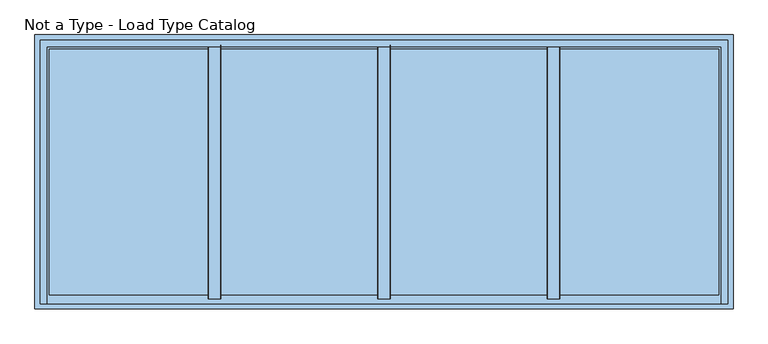
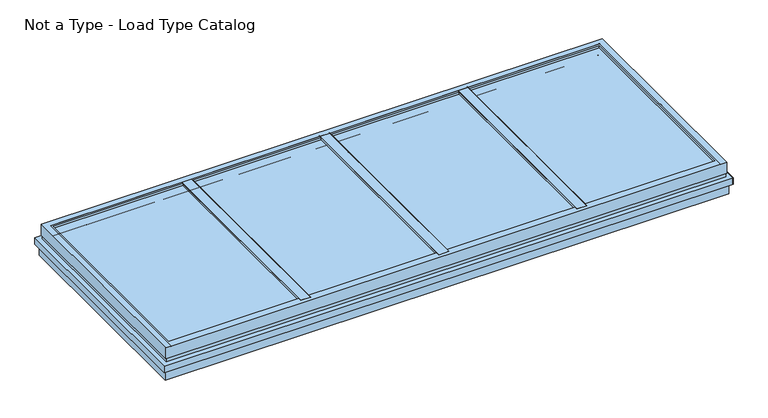
"""IFC4 building model written with IfcOpenShell, lengths in millimetres: window geometry, Skylight-Wasco-Low_Profile : Not a Type - Load Type Catalog."""

from ifc_helpers import new_model, si_unit, point, frame, frame_2d, origin, origin_with_axes, place, context, project, spatial, polyline, circle_curve, ellipse_curve, trimmed, segment, composite_curve, outline, extrude, source, transform, mapped, element, save
from ifc_brep_helpers import plane_surface, cylinder_surface, advanced_brep


def not_a_type_load_type_catalog_e0b292cc(model_context):
    return source(origin(), model_context, "Body", "SolidModel", [
        extrude(outline(composite_curve([segment(polyline([(192.3802188, 28.1940003), (192.3802188, -28.1940003)]), True, "CONTINUOUS"), segment(trimmed(circle_curve(frame_2d((178.9315699, -28.1940003)), 13.4486489), [point((192.3802188, -28.1940003))], [point((192.2262471, -30.2232155))], False, "CARTESIAN"), True, "CONTINUOUS"), segment(polyline([(192.2262471, -30.2232155), (179.4099406, -29.6347387), (179.4099406, -26.7462003), (176.2344841, -26.7462003), (176.2344841, -9.5227863), (142.8969841, -9.5227863), (142.8969841, -22.2249447), (139.7215663, -22.2249447), (139.7215663, -26.924), (138.1213663, -26.924), (136.5948503, -25.4), (111.715375, -25.4)]), True, "CONTINUOUS"), segment(trimmed(circle_curve(frame_2d((111.715375, -28.575)), 3.175), [point((111.715375, -25.4))], [point((108.5468841, -28.7782))], True, "CARTESIAN"), True, "CONTINUOUS"), segment(trimmed(circle_curve(frame_2d((111.715375, -28.9814)), 3.175), [point((108.5468841, -28.7782))], [point((111.715375, -32.1564))], True, "CARTESIAN"), True, "CONTINUOUS"), segment(polyline([(111.715375, -32.1564), (116.683615, -32.1564)]), True, "CONTINUOUS"), segment(trimmed(circle_curve(frame_2d((116.683615, -33.5407)), 1.3843), [point((116.683615, -32.1564))], [point((116.683615, -34.925))], False, "CARTESIAN"), True, "CONTINUOUS"), segment(polyline([(116.683615, -34.925), (101.6, -34.925), (101.6, 34.925), (116.683615, 34.925)]), True, "CONTINUOUS"), segment(trimmed(circle_curve(frame_2d((116.683615, 33.5407)), 1.3843), [point((116.683615, 34.925))], [point((116.683615, 32.1564))], False, "CARTESIAN"), True, "CONTINUOUS"), segment(polyline([(116.683615, 32.1564), (111.715375, 32.1564)]), True, "CONTINUOUS"), segment(trimmed(circle_curve(frame_2d((111.715375, 28.9814)), 3.175), [point((111.715375, 32.1564))], [point((108.5468841, 28.7782))], True, "CARTESIAN"), True, "CONTINUOUS"), segment(trimmed(circle_curve(frame_2d((111.715375, 28.575)), 3.175), [point((108.5468841, 28.7782))], [point((111.715375, 25.4))], True, "CARTESIAN"), True, "CONTINUOUS"), segment(polyline([(111.715375, 25.4), (136.5948503, 25.4), (138.1213663, 26.924), (139.7215663, 26.924), (139.7215663, 22.2249447), (142.8969841, 22.2249447), (142.8969841, 9.5227863), (176.2344841, 9.5227863), (176.2344841, 26.7462003), (179.4099406, 26.7462003), (179.4099406, 29.6347387), (190.2418721, 30.2232155)]), True, "CONTINUOUS"), segment(trimmed(circle_curve(frame_2d((190.3482188, 28.1940003)), 2.032), [point((190.2418721, 30.2232155))], [point((192.3802188, 28.1940003))], False, "CARTESIAN"), True, "CONTINUOUS")], self_intersect=False)), frame((0.0, -609.6, 0.0), z_axis=(0.0, 1.0, 0.0), x_axis=(0.0, 0.0, 1.0)), (0.0, 0.0, 1.0), 1219.2),
        extrude(outline(polyline([(25.4, -609.6), (-25.4, -609.6), (-25.4, 609.6), (25.4, 609.6), (25.4, -609.6)])), frame((0.0, 0.0, 0.3569904), z_axis=(0.0, 0.0, 1.0), x_axis=(1.0, 0.0, 0.0)), (0.0, 0.0, 1.0), 100.80625),
        extrude(outline(composite_curve([segment(polyline([(192.3802188, -784.6059997), (192.3802188, -840.9940003)]), True, "CONTINUOUS"), segment(trimmed(circle_curve(frame_2d((178.9315699, -840.9940003)), 13.4486489), [point((192.3802188, -840.9940003))], [point((192.2262471, -843.0232155))], False, "CARTESIAN"), True, "CONTINUOUS"), segment(polyline([(192.2262471, -843.0232155), (179.4099406, -842.4347387), (179.4099406, -839.5462003), (176.2344841, -839.5462003), (176.2344841, -822.3227863), (142.8969841, -822.3227863), (142.8969841, -835.0249447), (139.7215663, -835.0249447), (139.7215663, -839.724), (138.1213663, -839.724), (136.5948503, -838.2), (111.715375, -838.2)]), True, "CONTINUOUS"), segment(trimmed(circle_curve(frame_2d((111.715375, -841.375)), 3.175), [point((111.715375, -838.2))], [point((108.5468841, -841.5782))], True, "CARTESIAN"), True, "CONTINUOUS"), segment(trimmed(circle_curve(frame_2d((111.715375, -841.7814)), 3.175), [point((108.5468841, -841.5782))], [point((111.715375, -844.9564))], True, "CARTESIAN"), True, "CONTINUOUS"), segment(polyline([(111.715375, -844.9564), (116.683615, -844.9564)]), True, "CONTINUOUS"), segment(trimmed(circle_curve(frame_2d((116.683615, -846.3407)), 1.3843), [point((116.683615, -844.9564))], [point((116.683615, -847.725))], False, "CARTESIAN"), True, "CONTINUOUS"), segment(polyline([(116.683615, -847.725), (101.6, -847.725), (101.6, -777.875), (116.683615, -777.875)]), True, "CONTINUOUS"), segment(trimmed(circle_curve(frame_2d((116.683615, -779.2593)), 1.3843), [point((116.683615, -777.875))], [point((116.683615, -780.6436))], False, "CARTESIAN"), True, "CONTINUOUS"), segment(polyline([(116.683615, -780.6436), (111.715375, -780.6436)]), True, "CONTINUOUS"), segment(trimmed(circle_curve(frame_2d((111.715375, -783.8186)), 3.175), [point((111.715375, -780.6436))], [point((108.5468841, -784.0218))], True, "CARTESIAN"), True, "CONTINUOUS"), segment(trimmed(circle_curve(frame_2d((111.715375, -784.225)), 3.175), [point((108.5468841, -784.0218))], [point((111.715375, -787.4))], True, "CARTESIAN"), True, "CONTINUOUS"), segment(polyline([(111.715375, -787.4), (136.5948503, -787.4), (138.1213663, -785.876), (139.7215663, -785.876), (139.7215663, -790.5750553), (142.8969841, -790.5750553), (142.8969841, -803.2772137), (176.2344841, -803.2772137), (176.2344841, -786.0537997), (179.4099406, -786.0537997), (179.4099406, -783.1652613), (190.2418721, -782.5767845)]), True, "CONTINUOUS"), segment(trimmed(circle_curve(frame_2d((190.3482188, -784.6059997)), 2.032), [point((190.2418721, -782.5767845))], [point((192.3802188, -784.6059997))], False, "CARTESIAN"), True, "CONTINUOUS")], self_intersect=False)), frame((0.0, -609.6, 0.0), z_axis=(0.0, 1.0, 0.0), x_axis=(0.0, 0.0, 1.0)), (0.0, 0.0, 1.0), 1219.2),
        extrude(outline(polyline([(-787.4, -609.6), (-838.2, -609.6), (-838.2, 609.6), (-787.4, 609.6), (-787.4, -609.6)])), frame((0.0, 0.0, 0.3569904), z_axis=(0.0, 0.0, 1.0), x_axis=(1.0, 0.0, 0.0)), (0.0, 0.0, 1.0), 100.80625),
        extrude(outline(composite_curve([segment(polyline([(192.3802188, 840.9940003), (192.3802188, 784.6059997)]), True, "CONTINUOUS"), segment(trimmed(circle_curve(frame_2d((178.9315699, 784.6059997)), 13.4486489), [point((192.3802188, 784.6059997))], [point((192.2262471, 782.5767845))], False, "CARTESIAN"), True, "CONTINUOUS"), segment(polyline([(192.2262471, 782.5767845), (179.4099406, 783.1652613), (179.4099406, 786.0537997), (176.2344841, 786.0537997), (176.2344841, 803.2772137), (142.8969841, 803.2772137), (142.8969841, 790.5750553), (139.7215663, 790.5750553), (139.7215663, 785.876), (138.1213663, 785.876), (136.5948503, 787.4), (111.715375, 787.4)]), True, "CONTINUOUS"), segment(trimmed(circle_curve(frame_2d((111.715375, 784.225)), 3.175), [point((111.715375, 787.4))], [point((108.5468841, 784.0218))], True, "CARTESIAN"), True, "CONTINUOUS"), segment(trimmed(circle_curve(frame_2d((111.715375, 783.8186)), 3.175), [point((108.5468841, 784.0218))], [point((111.715375, 780.6436))], True, "CARTESIAN"), True, "CONTINUOUS"), segment(polyline([(111.715375, 780.6436), (116.683615, 780.6436)]), True, "CONTINUOUS"), segment(trimmed(circle_curve(frame_2d((116.683615, 779.2593)), 1.3843), [point((116.683615, 780.6436))], [point((116.683615, 777.875))], False, "CARTESIAN"), True, "CONTINUOUS"), segment(polyline([(116.683615, 777.875), (101.6, 777.875), (101.6, 847.725), (116.683615, 847.725)]), True, "CONTINUOUS"), segment(trimmed(circle_curve(frame_2d((116.683615, 846.3407)), 1.3843), [point((116.683615, 847.725))], [point((116.683615, 844.9564))], False, "CARTESIAN"), True, "CONTINUOUS"), segment(polyline([(116.683615, 844.9564), (111.715375, 844.9564)]), True, "CONTINUOUS"), segment(trimmed(circle_curve(frame_2d((111.715375, 841.7814)), 3.175), [point((111.715375, 844.9564))], [point((108.5468841, 841.5782))], True, "CARTESIAN"), True, "CONTINUOUS"), segment(trimmed(circle_curve(frame_2d((111.715375, 841.375)), 3.175), [point((108.5468841, 841.5782))], [point((111.715375, 838.2))], True, "CARTESIAN"), True, "CONTINUOUS"), segment(polyline([(111.715375, 838.2), (136.5948503, 838.2), (138.1213663, 839.724), (139.7215663, 839.724), (139.7215663, 835.0249447), (142.8969841, 835.0249447), (142.8969841, 822.3227863), (176.2344841, 822.3227863), (176.2344841, 839.5462003), (179.4099406, 839.5462003), (179.4099406, 842.4347387), (190.2418721, 843.0232155)]), True, "CONTINUOUS"), segment(trimmed(circle_curve(frame_2d((190.3482188, 840.9940003)), 2.032), [point((190.2418721, 843.0232155))], [point((192.3802188, 840.9940003))], False, "CARTESIAN"), True, "CONTINUOUS")], self_intersect=False)), frame((0.0, -609.6, 0.0), z_axis=(0.0, 1.0, 0.0), x_axis=(0.0, 0.0, 1.0)), (0.0, 0.0, 1.0), 1219.2),
        extrude(outline(polyline([(838.2, -609.6), (787.4, -609.6), (787.4, 609.6), (838.2, 609.6), (838.2, -609.6)])), frame((0.0, 0.0, 0.3569904), z_axis=(0.0, 0.0, 1.0), x_axis=(1.0, 0.0, 0.0)), (0.0, 0.0, 1.0), 100.80625),
        advanced_brep(
        [(-1603.6480651, -587.6480651, 136.468788), (-1607.2040651, -591.2040651, 132.912788), (-1607.2040651, 591.2040651, 132.912788), (-1603.6480651, 587.6480651, 136.468788), (-1603.6480651, 587.6480651, 146.0493661), (-1603.6480651, -587.6480651, 146.0493661), (-1617.109615, 601.109615, 192.469164), (-1617.109615, 601.109615, 193.8734375), (-1617.109615, -633.6302051, 193.8734375), (-1617.109615, -633.6302051, 192.469164), (-1594.8851432, -578.8851432, 117.475), (-1594.1231432, -578.1231432, 116.713), (-1594.1231432, 578.1231432, 116.713), (-1594.8851432, 578.8851432, 117.475), (-1672.1854051, -656.1854051, 101.6), (-1672.1854051, -656.1854051, 63.5), (-1672.1854051, 656.1854051, 63.5), (-1672.1854051, 656.1854051, 101.6), (-1674.2174051, -658.2174051, 63.5), (-1674.2174051, -658.2174051, 103.632), (-1674.2174051, 658.2174051, 103.632), (-1674.2174051, 658.2174051, 63.5), (-1606.55, -590.55, 192.469164), (-1606.55, -590.55, 179.3876533), (-1606.55, 590.55, 179.3876533), (-1606.55, 590.55, 192.469164), (-1622.3607127, -606.3607127, 179.3876533), (-1622.3607127, -606.3607127, 146.0493661), (-1622.3607127, 606.3607127, 146.0493661), (-1622.3607127, 606.3607127, 179.3876533), (-1612.3113821, -596.3113821, 132.912788), (-1612.3113821, -596.3113821, 117.475), (-1612.3113821, 596.3113821, 117.475), (-1612.3113821, 596.3113821, 132.912788), (-1594.1231432, -578.1231432, 101.6), (-1594.1231432, 578.1231432, 101.6), (-1646.4979432, -630.4979432, 103.632), (-1646.4979432, -630.4979432, 125.7990653), (-1646.4979432, 630.4979432, 125.7990653), (-1646.4979432, 630.4979432, 103.632), (-1649.6302051, -633.6302051, 125.7990653), (-1649.6302051, -633.6302051, 193.8734375), (-1649.6302051, 633.6302051, 193.8734375), (-1649.6302051, 633.6302051, 125.7990653), (1606.55, 590.55, 179.3876533), (1606.55, 590.55, 192.469164), (1622.3607127, 606.3607127, 146.0493661), (1622.3607127, 606.3607127, 179.3876533), (1612.3113821, 596.3113821, 117.475), (1612.3113821, 596.3113821, 132.912788), (1594.1231432, 578.1231432, 101.6), (1594.1231432, 578.1231432, 116.713), (1646.4979432, 630.4979432, 125.7990653), (1646.4979432, 630.4979432, 103.632), (1649.6302051, 633.6302051, 193.8734375), (1649.6302051, 633.6302051, 125.7990653), (1606.55, -590.55, 179.3876533), (1606.55, -590.55, 192.469164), (1622.3607127, -606.3607127, 146.0493661), (1622.3607127, -606.3607127, 179.3876533), (1612.3113821, -596.3113821, 117.475), (1612.3113821, -596.3113821, 132.912788), (1594.1231432, -578.1231432, 101.6), (1594.1231432, -578.1231432, 116.713), (1646.4979432, -630.4979432, 125.7990653), (1646.4979432, -630.4979432, 103.632), (1649.6302051, -633.6302051, 193.8734375), (1649.6302051, -633.6302051, 125.7990653), (1594.8851432, 578.8851432, 117.475), (1607.2040651, 591.2040651, 132.912788), (1603.6480651, 587.6480651, 136.468788), (1603.6480651, 587.6480651, 146.0493661), (1617.109615, 601.109615, 192.469164), (1617.109615, 601.109615, 193.8734375), (1594.8851432, -578.8851432, 117.475), (1607.2040651, -591.2040651, 132.912788), (1603.6480651, -587.6480651, 136.468788), (1603.6480651, -587.6480651, 146.0493661), (1617.109615, -633.6302051, 192.469164), (1617.109615, -633.6302051, 193.8734375), (1672.1854051, 656.1854051, 101.6), (1672.1854051, -656.1854051, 101.6), (1674.2174051, 658.2174051, 103.632), (1674.2174051, 658.2174051, 63.5), (1672.1854051, 656.1854051, 63.5), (1674.2174051, -658.2174051, 103.632), (1674.2174051, -658.2174051, 63.5), (1672.1854051, -656.1854051, 63.5)],
        [
            (0, 1, ellipse_curve(frame((-1607.2040651, -591.2040651, 136.468788), z_axis=(-0.7071067811865475, 0.7071067811865475, 0.0), x_axis=(-0.7071067811865474, -0.7071067811865476, 0.0)), 5.0289434, 3.556)),
            (1, 2),
            (2, 3, ellipse_curve(frame((-1607.2040651, 591.2040651, 136.468788), z_axis=(-0.7071067811865475, -0.7071067811865475, 0.0), x_axis=(0.7071067811865474, -0.7071067811865476, 0.0)), 5.0289434, 3.556)),
            (3, 0),
            (3, 4),
            (4, 5),
            (5, 0),
            (6, 7),
            (7, 8),
            (8, 9),
            (9, 6),
            (10, 11, ellipse_curve(frame((-1594.8851432, -578.8851432, 116.713), z_axis=(-0.7071067811865475, 0.7071067811865475, 0.0), x_axis=(-0.7071067811865474, -0.7071067811865476, 0.0)), 1.0776307, 0.762)),
            (11, 12),
            (12, 13, ellipse_curve(frame((-1594.8851432, 578.8851432, 116.713), z_axis=(-0.7071067811865475, -0.7071067811865475, 0.0), x_axis=(0.7071067811865474, -0.7071067811865476, 0.0)), 1.0776307, 0.762)),
            (13, 10),
            (14, 15),
            (15, 16),
            (16, 17),
            (17, 14),
            (18, 19),
            (19, 20),
            (20, 21),
            (21, 18),
            (22, 23),
            (23, 24),
            (24, 25),
            (25, 22),
            (26, 27),
            (27, 28),
            (28, 29),
            (29, 26),
            (30, 31),
            (31, 32),
            (32, 33),
            (33, 30),
            (11, 34),
            (34, 35),
            (35, 12),
            (36, 37),
            (37, 38),
            (38, 39),
            (39, 36),
            (40, 41),
            (41, 42),
            (42, 43),
            (43, 40),
            (24, 44),
            (44, 45),
            (45, 25),
            (28, 46),
            (46, 47),
            (47, 29),
            (32, 48),
            (48, 49),
            (49, 33),
            (35, 50),
            (50, 51),
            (51, 12),
            (38, 52),
            (52, 53),
            (53, 39),
            (42, 54),
            (54, 55),
            (55, 43),
            (44, 56),
            (56, 57),
            (57, 45),
            (46, 58),
            (58, 59),
            (59, 47),
            (48, 60),
            (60, 61),
            (61, 49),
            (50, 62),
            (62, 63),
            (63, 51),
            (52, 64),
            (64, 65),
            (65, 53),
            (54, 66),
            (66, 67),
            (67, 55),
            (51, 68, ellipse_curve(frame((1594.8851432, 578.8851432, 116.713), z_axis=(-0.7071067811865475, 0.7071067811865475, 0.0), x_axis=(-0.7071067811865476, -0.7071067811865474, 0.0)), 1.0776307, 0.762)),
            (68, 13),
            (2, 69),
            (69, 70, ellipse_curve(frame((1607.2040651, 591.2040651, 136.468788), z_axis=(-0.7071067811865475, 0.7071067811865475, 0.0), x_axis=(-0.7071067811865476, -0.7071067811865474, 0.0)), 5.0289434, 3.556)),
            (70, 3),
            (70, 71),
            (71, 4),
            (6, 72),
            (72, 73),
            (73, 7),
            (63, 74, ellipse_curve(frame((1594.8851432, -578.8851432, 116.713), z_axis=(0.7071067811865475, 0.7071067811865475, 0.0), x_axis=(-0.7071067811865474, 0.7071067811865476, 0.0)), 1.0776307, 0.762)),
            (74, 68),
            (69, 75),
            (75, 76, ellipse_curve(frame((1607.2040651, -591.2040651, 136.468788), z_axis=(0.7071067811865475, 0.7071067811865475, 0.0), x_axis=(-0.7071067811865474, 0.7071067811865476, 0.0)), 5.0289434, 3.556)),
            (76, 70),
            (76, 77),
            (77, 71),
            (72, 78),
            (78, 79),
            (79, 73),
            (40, 67),
            (66, 79),
            (78, 9),
            (8, 41),
            (37, 64),
            (36, 65),
            (17, 80),
            (80, 81),
            (81, 14),
            (34, 62),
            (11, 63),
            (10, 74),
            (31, 60),
            (30, 61),
            (1, 75),
            (0, 76),
            (5, 77),
            (27, 58),
            (26, 59),
            (23, 56),
            (57, 22),
            (20, 82),
            (82, 83),
            (83, 21),
            (16, 84),
            (84, 80),
            (82, 85),
            (85, 86),
            (86, 83),
            (84, 87),
            (87, 81),
            (19, 85),
            (18, 86),
            (15, 87),
        ],
        [
            cylinder_surface(frame((-1607.2040651, -633.6302051, 136.468788), z_axis=(0.0, -1.0, 0.0), x_axis=(1.0, 0.0, 0.0)), 3.556),
            plane_surface(frame((-1603.6480651, -587.6480651, 136.468788), z_axis=(1.0, 0.0, 0.0), x_axis=(0.0, 1.0, 0.0))),
            plane_surface(frame((-1617.109615, -601.109615, 192.469164), z_axis=(1.0, 0.0, 0.0), x_axis=(0.0, 1.0, 0.0))),
            cylinder_surface(frame((-1594.8851432, -633.6302051, 116.713), z_axis=(0.0, -1.0, 0.0), x_axis=(1.0, 0.0, 0.0)), 0.762),
            plane_surface(frame((-1672.1854051, -656.1854051, 63.5), z_axis=(1.0, 0.0, 0.0), x_axis=(0.0, 1.0, 0.0))),
            plane_surface(frame((-1674.2174051, -658.2174051, 103.632), z_axis=(-1.0, 0.0, 0.0), x_axis=(0.0, 1.0, 0.0))),
            plane_surface(frame((-1606.55, -590.55, 179.3876533), z_axis=(1.0, 0.0, 0.0), x_axis=(0.0, 1.0, 0.0))),
            plane_surface(frame((-1622.3607127, -606.3607127, 146.0493661), z_axis=(1.0, 0.0, 0.0), x_axis=(0.0, 1.0, 0.0))),
            plane_surface(frame((-1612.3113821, -596.3113821, 117.475), z_axis=(1.0, 0.0, 0.0), x_axis=(0.0, 1.0, 0.0))),
            plane_surface(frame((-1594.1231432, -578.1231432, 101.6), z_axis=(1.0, 0.0, 0.0), x_axis=(0.0, 1.0, 0.0))),
            plane_surface(frame((-1646.4979432, -630.4979432, 125.7990653), z_axis=(-1.0, 0.0, 0.0), x_axis=(0.0, 1.0, 0.0))),
            plane_surface(frame((-1649.6302051, -633.6302051, 193.8734375), z_axis=(-1.0, 0.0, 0.0), x_axis=(0.0, 1.0, 0.0))),
            plane_surface(frame((-1606.55, 590.55, 179.3876533), z_axis=(0.0, -1.0, 0.0), x_axis=(1.0, 0.0, 0.0))),
            plane_surface(frame((-1622.3607127, 606.3607127, 146.0493661), z_axis=(0.0, -1.0, 0.0), x_axis=(1.0, 0.0, 0.0))),
            plane_surface(frame((-1612.3113821, 596.3113821, 117.475), z_axis=(0.0, -1.0, 0.0), x_axis=(1.0, 0.0, 0.0))),
            plane_surface(frame((-1594.1231432, 578.1231432, 101.6), z_axis=(0.0, -1.0, 0.0), x_axis=(1.0, 0.0, 0.0))),
            plane_surface(frame((-1646.4979432, 630.4979432, 125.7990653), z_axis=(0.0, 1.0, 0.0), x_axis=(1.0, 0.0, 0.0))),
            plane_surface(frame((-1649.6302051, 633.6302051, 193.8734375), z_axis=(0.0, 1.0, 0.0), x_axis=(1.0, 0.0, 0.0))),
            plane_surface(frame((1606.55, 590.55, 179.3876533), z_axis=(-1.0, 0.0, 0.0), x_axis=(0.0, -1.0, 0.0))),
            plane_surface(frame((1622.3607127, 606.3607127, 146.0493661), z_axis=(-1.0, 0.0, 0.0), x_axis=(0.0, -1.0, 0.0))),
            plane_surface(frame((1612.3113821, 596.3113821, 117.475), z_axis=(-1.0, 0.0, 0.0), x_axis=(0.0, -1.0, 0.0))),
            plane_surface(frame((1594.1231432, 578.1231432, 101.6), z_axis=(-1.0, 0.0, 0.0), x_axis=(0.0, -1.0, 0.0))),
            plane_surface(frame((1646.4979432, 630.4979432, 125.7990653), z_axis=(1.0, 0.0, 0.0), x_axis=(0.0, -1.0, 0.0))),
            plane_surface(frame((1649.6302051, 633.6302051, 193.8734375), z_axis=(1.0, 0.0, 0.0), x_axis=(0.0, -1.0, 0.0))),
            cylinder_surface(frame((-1649.6302051, 578.8851432, 116.713), z_axis=(-1.0, 0.0, 0.0), x_axis=(0.0, -1.0, 0.0)), 0.762),
            cylinder_surface(frame((-1649.6302051, 591.2040651, 136.468788), z_axis=(-1.0, 0.0, 0.0), x_axis=(0.0, -1.0, 0.0)), 3.556),
            plane_surface(frame((-1603.6480651, 587.6480651, 136.468788), z_axis=(0.0, -1.0, 0.0), x_axis=(1.0, 0.0, 0.0))),
            plane_surface(frame((-1617.109615, 601.109615, 192.469164), z_axis=(0.0, -1.0, 0.0), x_axis=(1.0, 0.0, 0.0))),
            cylinder_surface(frame((1594.8851432, 633.6302051, 116.713), z_axis=(0.0, 1.0, 0.0), x_axis=(-1.0, 0.0, 0.0)), 0.762),
            cylinder_surface(frame((1607.2040651, 633.6302051, 136.468788), z_axis=(0.0, 1.0, 0.0), x_axis=(-1.0, 0.0, 0.0)), 3.556),
            plane_surface(frame((1603.6480651, 587.6480651, 136.468788), z_axis=(-1.0, 0.0, 0.0), x_axis=(0.0, -1.0, 0.0))),
            plane_surface(frame((1617.109615, 601.109615, 192.469164), z_axis=(-1.0, 0.0, 0.0), x_axis=(0.0, -1.0, 0.0))),
            plane_surface(frame((1649.6302051, -633.6302051, 193.8734375), z_axis=(0.0, -1.0, 0.0), x_axis=(-1.0, 0.0, 0.0))),
            plane_surface(frame((1649.6302051, -633.6302051, 125.7990653), z_axis=(0.0, 0.0, -1.0), x_axis=(-1.0, 0.0, 0.0))),
            plane_surface(frame((1646.4979432, -630.4979432, 125.7990653), z_axis=(0.0, -1.0, 0.0), x_axis=(-1.0, 0.0, 0.0))),
            plane_surface(frame((1672.1854051, -656.1854051, 101.6), z_axis=(0.0, 0.0, -1.0), x_axis=(-1.0, 0.0, 0.0))),
            plane_surface(frame((1594.1231432, -578.1231432, 101.6), z_axis=(0.0, 1.0, 0.0), x_axis=(-1.0, 0.0, 0.0))),
            cylinder_surface(frame((1649.6302051, -578.8851432, 116.713), z_axis=(1.0, 0.0, 0.0), x_axis=(0.0, 1.0, 0.0)), 0.762),
            plane_surface(frame((1594.8851432, -578.8851432, 117.475), z_axis=(0.0, 0.0, 1.0), x_axis=(-1.0, 0.0, 0.0))),
            plane_surface(frame((1612.3113821, -596.3113821, 117.475), z_axis=(0.0, 1.0, 0.0), x_axis=(-1.0, 0.0, 0.0))),
            plane_surface(frame((1612.3113821, -596.3113821, 132.912788), z_axis=(0.0, 0.0, -1.0), x_axis=(-1.0, 0.0, 0.0))),
            cylinder_surface(frame((1649.6302051, -591.2040651, 136.468788), z_axis=(1.0, 0.0, 0.0), x_axis=(0.0, 1.0, 0.0)), 3.556),
            plane_surface(frame((1603.6480651, -587.6480651, 136.468788), z_axis=(0.0, 1.0, 0.0), x_axis=(-1.0, 0.0, 0.0))),
            plane_surface(frame((1603.6480651, -587.6480651, 146.0493661), z_axis=(0.0, 0.0, 1.0), x_axis=(-1.0, 0.0, 0.0))),
            plane_surface(frame((1622.3607127, -606.3607127, 146.0493661), z_axis=(0.0, 1.0, 0.0), x_axis=(-1.0, 0.0, 0.0))),
            plane_surface(frame((1622.3607127, -606.3607127, 179.3876533), z_axis=(0.0, 0.0, -1.0), x_axis=(-1.0, 0.0, 0.0))),
            plane_surface(frame((1606.55, -590.55, 192.469164), z_axis=(0.0, 0.0, 1.0), x_axis=(-1.0, 0.0, 0.0))),
            plane_surface(frame((1617.109615, -601.109615, 193.8734375), z_axis=(0.0, 0.0, 1.0), x_axis=(-1.0, 0.0, 0.0))),
            plane_surface(frame((-1674.2174051, 658.2174051, 103.632), z_axis=(0.0, 1.0, 0.0), x_axis=(1.0, 0.0, 0.0))),
            plane_surface(frame((-1672.1854051, 656.1854051, 63.5), z_axis=(0.0, -1.0, 0.0), x_axis=(1.0, 0.0, 0.0))),
            plane_surface(frame((1674.2174051, 658.2174051, 103.632), z_axis=(1.0, 0.0, 0.0), x_axis=(0.0, -1.0, 0.0))),
            plane_surface(frame((1672.1854051, 656.1854051, 63.5), z_axis=(-1.0, 0.0, 0.0), x_axis=(0.0, -1.0, 0.0))),
            plane_surface(frame((1646.4979432, -630.4979432, 103.632), z_axis=(0.0, 0.0, 1.0), x_axis=(-1.0, 0.0, 0.0))),
            plane_surface(frame((1674.2174051, -658.2174051, 103.632), z_axis=(0.0, -1.0, 0.0), x_axis=(-1.0, 0.0, 0.0))),
            plane_surface(frame((1674.2174051, -658.2174051, 63.5), z_axis=(0.0, 0.0, -1.0), x_axis=(-1.0, 0.0, 0.0))),
            plane_surface(frame((1672.1854051, -656.1854051, 63.5), z_axis=(0.0, 1.0, 0.0), x_axis=(-1.0, 0.0, 0.0))),
            plane_surface(frame((1606.55, -590.55, 179.3876533), z_axis=(0.0, 1.0, 0.0), x_axis=(-1.0, 0.0, 0.0))),
        ],
        [
            (0, [[1, 2, 3, 4]]),
            (1, [[-4, 5, 6, 7]]),
            (2, [[8, 9, 10, 11]]),
            (3, [[12, 13, 14, 15]]),
            (4, [[16, 17, 18, 19]]),
            (5, [[20, 21, 22, 23]]),
            (6, [[24, 25, 26, 27]]),
            (7, [[28, 29, 30, 31]]),
            (8, [[32, 33, 34, 35]]),
            (9, [[-13, 36, 37, 38]]),
            (10, [[39, 40, 41, 42]]),
            (11, [[43, 44, 45, 46]]),
            (12, [[-26, 47, 48, 49]]),
            (13, [[-30, 50, 51, 52]]),
            (14, [[-34, 53, 54, 55]]),
            (15, [[-38, 56, 57, 58]]),
            (16, [[-41, 59, 60, 61]]),
            (17, [[-45, 62, 63, 64]]),
            (18, [[-48, 65, 66, 67]]),
            (19, [[-51, 68, 69, 70]]),
            (20, [[-54, 71, 72, 73]]),
            (21, [[-57, 74, 75, 76]]),
            (22, [[-60, 77, 78, 79]]),
            (23, [[-63, 80, 81, 82]]),
            (24, [[-14, -58, 83, 84]]),
            (25, [[-3, 85, 86, 87]]),
            (26, [[-5, -87, 88, 89]]),
            (27, [[-8, 90, 91, 92]]),
            (28, [[-76, 93, 94, -83]]),
            (29, [[-86, 95, 96, 97]]),
            (30, [[-88, -97, 98, 99]]),
            (31, [[-91, 100, 101, 102]]),
            (32, [[-43, 103, -81, 104, -101, 105, -10, 106]]),
            (33, [[-46, -64, -82, -103], [-40, 107, -77, -59]]),
            (34, [[-39, 108, -78, -107]]),
            (35, [[-19, 109, 110, 111], [-37, 112, -74, -56]]),
            (36, [[-36, 113, -75, -112]]),
            (37, [[-12, 114, -93, -113]]),
            (38, [[-33, 115, -71, -53], [-15, -84, -94, -114]]),
            (39, [[-32, 116, -72, -115]]),
            (40, [[-35, -55, -73, -116], [-2, 117, -95, -85]]),
            (41, [[-1, 118, -96, -117]]),
            (42, [[-7, 119, -98, -118]]),
            (43, [[-29, 120, -68, -50], [-6, -89, -99, -119]]),
            (44, [[-28, 121, -69, -120]]),
            (45, [[-31, -52, -70, -121], [-25, 122, -65, -47]]),
            (46, [[-100, -90, -11, -105], [-27, -49, -67, 123]]),
            (47, [[-44, -106, -9, -92, -102, -104, -80, -62]]),
            (48, [[-22, 124, 125, 126]]),
            (49, [[-18, 127, 128, -109]]),
            (50, [[-125, 129, 130, 131]]),
            (51, [[-110, -128, 132, 133]]),
            (52, [[-21, 134, -129, -124], [-42, -61, -79, -108]]),
            (53, [[-20, 135, -130, -134]]),
            (54, [[-23, -126, -131, -135], [-17, 136, -132, -127]]),
            (55, [[-16, -111, -133, -136]]),
            (56, [[-24, -123, -66, -122]]),
        ],
    ),
        extrude(outline(polyline([(-1622.3607127, -629.7041932), (-1622.3607127, 606.3607127), (1622.3607127, 606.3607127), (1622.3607127, -629.7041932), (-1622.3607127, -629.7041932)])), frame((0.0, 0.0, 139.6799684), z_axis=(0.0, 0.0, 1.0), x_axis=(1.0, 0.0, 0.0)), (0.0, 0.0, 1.0), 33.3375),
        extrude(outline(polyline([(1657.35, 641.35), (1657.35, -641.35), (-1657.35, -641.35), (-1657.35, 641.35), (1657.35, 641.35)]), holes=[polyline([(1606.55, 590.55), (-1606.55, 590.55), (-1606.55, -590.55), (1606.55, -590.55), (1606.55, 590.55)])]), origin_with_axes(), (0.0, 0.0, 1.0), 101.6),
    ])


if __name__ == "__main__":
    model = new_model("IFC4")
    model_context = context("Model", 3, world=origin())
    ifc_project = project(units=[si_unit("LENGTHUNIT", "METRE", prefix="MILLI")], contexts=[model_context])
    site = spatial("IfcSite", under=ifc_project)
    building = spatial("IfcBuilding", under=site)
    placement = place(None, origin())
    not_a_type_load_type_catalog_shape = not_a_type_load_type_catalog_e0b292cc(model_context)
    element("IfcWindow", 1, ObjectType="Skylight-Wasco-Low_Profile : Not a Type - Load Type Catalog", at=placement, inside=building, context=model_context, shape_type="MappedRepresentation", body=[
        mapped(not_a_type_load_type_catalog_shape, transform((0.0, 0.0, 0.0), x_axis=(1.0, 0.0, 0.0), y_axis=(0.0, 1.0, 0.0), z_axis=(0.0, 0.0, 1.0))),
    ])
    save(model, "model.ifc")

# Revit data of these elements
# Type "Skylight-Wasco-Low_Profile : Not a Type - Load Type Catalog"
#   Type Mark = "15"
#   URL = "http://www.wascoskylights.com/"
#   Product Page URL = "http://www.wascoskylights.com/commercial/configurations/glass/low-profile"
#   Product Name = "Low Profile"
#   Product Documentation Link = "http://www.wascoskylights.com/commercial/products/pinnacle350"
#   Model = "LPGS-12848"
#   Material = ""
#   Manufacturer = "Wasco"
#   Description = "Skylight"
#   Width = 4' - 1 1/2"
#   Support Width [instance default] = 0' - 2"
#   Support Height [instance default] = 0' - 3 23/32"
#   Rough Width = 3' - 10 1/2"
#   Rough Length = 10' - 6 1/2"
#   Rough Height = 0' - 7 81/128"
#   Purling Array Offset [instance default] = 2' - 0"
#   Mounting Height [instance default] = 0' - 4"
#   Length = 10' - 9 1/2"
#   Host Width = 6' - 1 1/2"
#   Host Length = 12' - 9 1/2"
#   Height = 0' - 3 81/128"
#   Curb Width = 0' - 2"
#   Curb Height = 0' - 4"
#   C Curb Width [instance default] = 0' - 2"
#   Rafter Array = 3
#   Purlin [instance default] = no
#   Number of Purlins [instance default] = 5
#   Host Constraint = 1
#   Glazing 1 5_16 = yes
#   Glazing 1 3_16 = no
#   Glazing 1 1_16 = no
#   Deck Mount = no
#   Curb Mount = yes
#   2' Rafter Spacing = no
#   1' 4" Rafter Spacing = yes
#   Glazing Material = Glass - Wasco - Clear
#   Finish = Aluminum - Wasco - Aged Copper
#   Curb = Rubber, Black
#   Default Elevation = 0
# Element 1 (IfcWindow, "Skylight-Wasco-Low_Profile : Not a Type - Load Type Catalog")
#   Materials on its faces: "Aluminum - Wasco - Aged Copper", "Rubber, Black", "Glass - Wasco - Clear"
# Materials
#   "Glass - Wasco - Clear": class "Glass", colour RGB 218 227 224, transparency 0.85, Description = "Clear glazing", Cost = 0
#   "Aluminum - Wasco - Aged Copper": class "Metal", colour RGB 125 165 130, transparency 0, Description = "Aluminum 6061", Cost = 0
#   "Rubber, Black": class "Plastic", colour RGB 63 63 63, transparency 0, Description = "Natural rubber, black", Cost = 0
